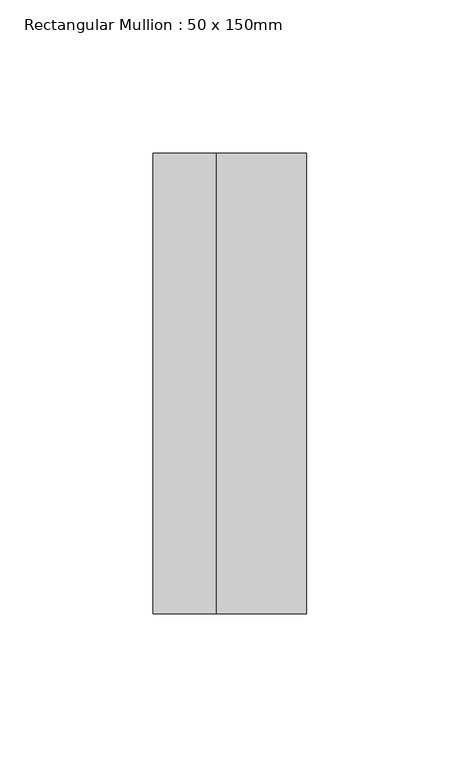
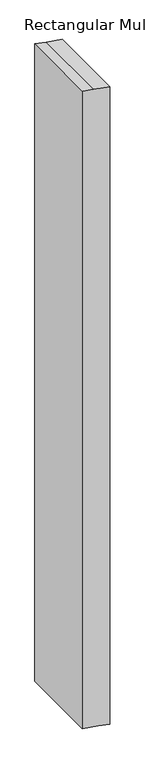
"""IFC4 building model written with IfcOpenShell, lengths in millimetres: member geometry, Rectangular Mullion : 50 x 150mm."""

from ifc_helpers import new_model, si_unit, frame, origin, place, context, project, spatial, polyline, outline, extrude, source, transform, mapped, element, save


def rectangular_mullion_50_x_150mm_4beb3cf6(model_context):
    return source(origin(), model_context, "Body", "SweptSolid", [
        extrude(outline(polyline([(-4.7938398, 25.0), (0.3798062, -4.3412044), (4.0225092, -25.0), (-1227.3293292, -25.0), (-1232.5029752, 4.3412044), (-1236.1456782, 25.0), (-4.7938398, 25.0)])), frame((0.0, -75.0, 0.0), z_axis=(0.0, 1.0, 0.0), x_axis=(0.0, 0.0, 1.0)), (0.0, 0.0, 1.0), 150.0),
    ])


if __name__ == "__main__":
    model = new_model("IFC4")
    model_context = context("Model", 3, world=origin())
    ifc_project = project(units=[si_unit("LENGTHUNIT", "METRE", prefix="MILLI")], contexts=[model_context])
    site = spatial("IfcSite", under=ifc_project)
    building = spatial("IfcBuilding", under=site)
    placement = place(None, origin())
    rectangular_mullion_50_x_150mm_shape = rectangular_mullion_50_x_150mm_4beb3cf6(model_context)
    element("IfcMember", 1, ObjectType="Rectangular Mullion : 50 x 150mm", at=placement, inside=building, context=model_context, shape_type="MappedRepresentation", body=[
        mapped(rectangular_mullion_50_x_150mm_shape, transform((0.0, 0.0, 0.0), x_axis=(1.0, 0.0, 0.0), y_axis=(0.0, 1.0, 0.0), z_axis=(0.0, 0.0, 1.0))),
    ])
    save(model, "model.ifc")

# Revit data of these elements
# Type "Rectangular Mullion : 50 x 150mm"
#   built-in parameter 1007304 = 0.492126 (stored number, unit not read)
#   built-in parameter 1007301 = 0.082021 (stored number, unit not read)
#   built-in parameter 1007300 = 0.082021 (stored number, unit not read)
# Element 1 (IfcMember, "Rectangular Mullion : 50 x 150mm")
#   Materials on its faces: "Aluminium"
# Materials
#   "Aluminium": class "Metal", colour RGB 247 247 247, transparency 0, Description = "Aluminium 6061", Cost = 0
